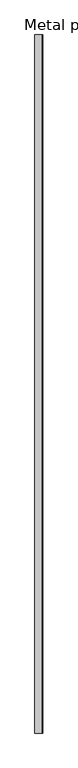
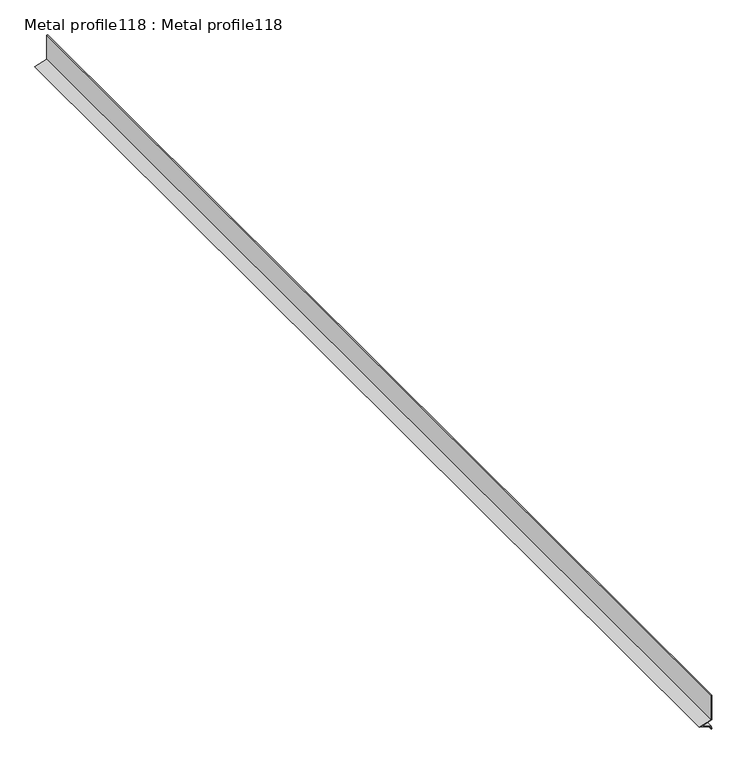
"""IFC4 building model written with IfcOpenShell, lengths in millimetres: proxy geometry, Metal profile118 : Metal profile118."""

from ifc_helpers import new_model, si_unit, frame, origin, place, context, project, spatial, polyline, outline, extrude, source, transform, mapped, element, save


def metal_profile118_metal_profile118_c184cb36(model_context):
    return source(origin(), model_context, "Body", "SweptSolid", [
        extrude(outline(polyline([(39099.4100034, 10041.7862048), (39104.5247538, 10040.8230098), (39110.0249118, 10023.7114071), (39115.8346682, 10041.7862048), (39160.8249118, 10041.7862048), (39160.8249118, 10040.5162048), (39116.7604475, 10040.5162048), (39110.0249118, 10019.5612048), (39103.5469636, 10039.7148214), (39099.1749719, 10040.5381423), (39099.4100034, 10041.7862048)])), frame((0.0, 2217.3611963, 0.0), z_axis=(0.0, 1.0, 0.0), x_axis=(0.0, 0.0, 1.0)), (0.0, 0.0, 1.0), 2000.0),
    ])


if __name__ == "__main__":
    model = new_model("IFC4")
    model_context = context("Model", 3, world=origin())
    ifc_project = project(units=[si_unit("LENGTHUNIT", "METRE", prefix="MILLI")], contexts=[model_context])
    site = spatial("IfcSite", under=ifc_project)
    building = spatial("IfcBuilding", under=site)
    placement = place(None, origin())
    metal_profile118_metal_profile118_shape = metal_profile118_metal_profile118_c184cb36(model_context)
    element("IfcBuildingElementProxy", 1, Name="Metal profile118 : Metal profile118", ObjectType="Metal profile118 : Metal profile118", at=placement, inside=building, context=model_context, shape_type="MappedRepresentation", body=[
        mapped(metal_profile118_metal_profile118_shape, transform((0.0, 0.0, 0.0), x_axis=(1.0, 0.0, 0.0), y_axis=(0.0, 1.0, 0.0), z_axis=(0.0, 0.0, 1.0))),
    ])
    save(model, "model.ifc")

# Revit data of these elements
# Type "Metal profile118 : Metal profile118"
#   NameOverride = "Metal profile118"
# Element 1 (IfcBuildingElementProxy, "Metal profile118 : Metal profile118")
#   Materials on its faces: "16 GA. COPPER WEEP SCREED W/ MIN 3 1/2\" ATTACHMENT FLANGE - LAP UNDERLAYMENT OVER WEED SCREED"
# Materials
#   "16 GA. COPPER WEEP SCREED W/ MIN 3 1/2\" ATTACHMENT FLANGE - LAP UNDERLAYMENT OVER WEED SCREED": class "Unassigned", colour RGB 251 232 155, transparency 0, Cost = 0
